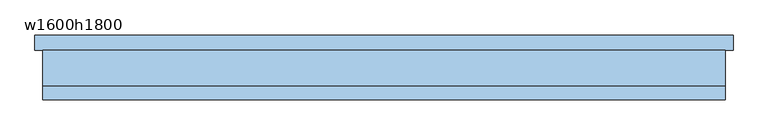
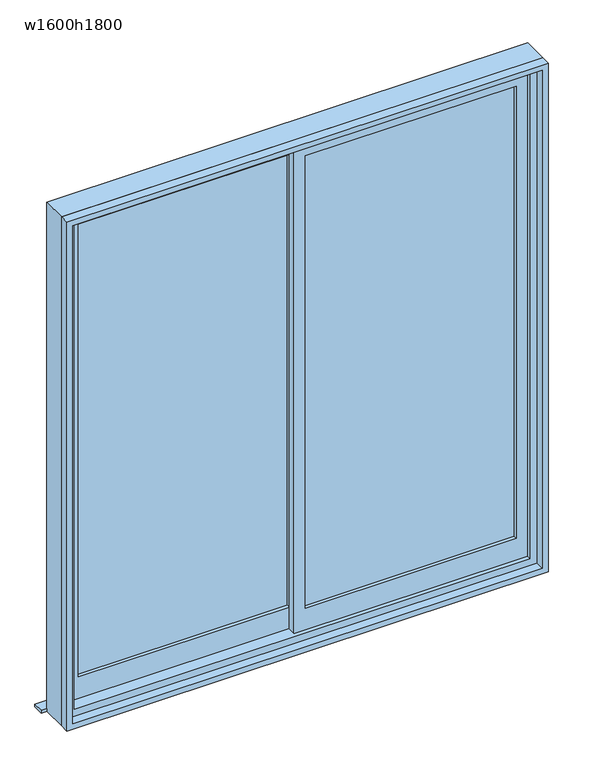
"""IFC4 building model written with IfcOpenShell, lengths in millimetres: window geometry, 引違い掃出窓_2枚 : w1600h1800."""

from ifc_helpers import new_model, si_unit, frame, origin, place, context, project, spatial, polyline, outline, extrude, source, transform, mapped, element, save


def w1600h1800_0506f16c(model_context):
    return source(origin(), model_context, "Body", "SweptSolid", [
        extrude(outline(polyline([(-20.0, 12.5), (-760.0, 12.5), (-760.0, 17.5), (-20.0, 17.5), (-20.0, 12.5)])), frame((0.0, 0.0, 280.0), z_axis=(0.0, 0.0, 1.0), x_axis=(1.0, 0.0, 0.0)), (0.0, 0.0, 1.0), 1680.0),
        extrude(outline(polyline([(760.0, -17.5), (20.0, -17.5), (20.0, -12.5), (760.0, -12.5), (760.0, -17.5)])), frame((0.0, 0.0, 280.0), z_axis=(0.0, 0.0, 1.0), x_axis=(1.0, 0.0, 0.0)), (0.0, 0.0, 1.0), 1680.0),
        extrude(outline(polyline([(2000.0, -20.0), (200.0, -20.0), (200.0, 800.0), (2000.0, 800.0), (2000.0, -20.0)]), holes=[polyline([(280.0, 760.0), (280.0, 20.0), (1960.0, 20.0), (1960.0, 760.0), (280.0, 760.0)])]), frame((0.0, -30.0, 0.0), z_axis=(0.0, 1.0, 0.0), x_axis=(0.0, 0.0, 1.0)), (0.0, 0.0, 1.0), 30.0),
        extrude(outline(polyline([(2000.0, -800.0), (200.0, -800.0), (200.0, 20.0), (2000.0, 20.0), (2000.0, -800.0)]), holes=[polyline([(280.0, -20.0), (280.0, -760.0), (1960.0, -760.0), (1960.0, -20.0), (280.0, -20.0)])]), frame((0.0, 0.0, 0.0), z_axis=(0.0, 1.0, 0.0), x_axis=(0.0, 0.0, 1.0)), (0.0, 0.0, 1.0), 30.0),
        extrude(outline(polyline([(865.0, 82.75), (865.0, 45.0), (-865.0, 45.0), (-865.0, 82.75), (865.0, 82.75)])), frame((0.0, 0.0, 155.0), z_axis=(0.0, 0.0, 1.0), x_axis=(1.0, 0.0, 0.0)), (0.0, 0.0, 1.0), 10.0),
        extrude(outline(polyline([(2045.0, 845.0), (2045.0, -845.0), (155.0, -845.0), (155.0, 845.0), (2045.0, 845.0)]), holes=[polyline([(175.0, -825.0), (2025.0, -825.0), (2025.0, 825.0), (175.0, 825.0), (175.0, -825.0)])]), frame((0.0, -77.75, 0.0), z_axis=(0.0, 1.0, 0.0), x_axis=(0.0, 0.0, 1.0)), (0.0, 0.0, 1.0), 32.75),
        extrude(outline(polyline([(2045.0, -845.0), (155.0, -845.0), (155.0, 845.0), (2045.0, 845.0), (2045.0, -845.0)]), holes=[polyline([(2000.0, 800.0), (200.0, 800.0), (200.0, -800.0), (2000.0, -800.0), (2000.0, 800.0)])]), frame((0.0, -45.0, 0.0), z_axis=(0.0, 1.0, 0.0), x_axis=(0.0, 0.0, 1.0)), (0.0, 0.0, 1.0), 90.0),
    ])


if __name__ == "__main__":
    model = new_model("IFC4")
    model_context = context("Model", 3, world=origin())
    ifc_project = project(units=[si_unit("LENGTHUNIT", "METRE", prefix="MILLI")], contexts=[model_context])
    site = spatial("IfcSite", under=ifc_project)
    building = spatial("IfcBuilding", under=site)
    placement = place(None, origin())
    w1600h1800_shape = w1600h1800_0506f16c(model_context)
    element("IfcWindow", 1, ObjectType="引違い掃出窓_2枚 : w1600h1800", at=placement, inside=building, context=model_context, shape_type="MappedRepresentation", body=[
        mapped(w1600h1800_shape, transform((0.0, 0.0, 0.0), x_axis=(1.0, 0.0, 0.0), y_axis=(0.0, 1.0, 0.0), z_axis=(0.0, 0.0, 1.0))),
    ])
    save(model, "model.ifc")

# Revit data of these elements
# Project information
#   プロジェクト発行日 = "発行日"
#   プロジェクト ステータス = "プロジェクト ステータス"
#   クライアント名 = "オーナ"
#   計画地住所 = "ここにアドレスを入力"
#   プロジェクト名 = "プロジェクト名"
#   プロジェクト番号 = "0001"
# Type "引違い掃出窓_2枚 : w1600h1800"
#   Construction Type Id = "GSP4R"
#   Analytic Construction = "1/8 インチ ピルキントン一重ガラス"
#   Type Mark = "67"
#   Operation = "ダブル パネル縦"
#   Keynote = "08520.R1"
#   Visual Light Transmittance = 0.9
#   Solar Heat Gain Coefficient = 0.86
#   Heat Transfer Coefficient (U) = 6.7069 W/(m²·K)
#   Height = 1800 mm
#   既定の腰高 = 200 mm
#   Width = 1600 mm
#   額縁見附 = 20 mm
#   額縁ちり = 10 mm
#   サッシ見附 = 45 mm
#   サッシの幅 = 90 mm
#   サッシ額縁 [instance default] = none
#   サッシ本体 [instance default] = none
#   サッシガラス [instance default] = ガラス - 透明
#   Manufacturer = ""
#   Wall Closure = (empty or 0)
#   Model = ""
#   Type Comments = ""
#   Assembly Code = ""
# Element 1 (IfcWindow, "引違い掃出窓_2枚 : w1600h1800")
#   Materials on its faces: "ガラス - 透明"
# Materials
#   "ガラス - 透明": class "ガラス", colour RGB 0 128 192, transparency 0.9, Cost = 0
